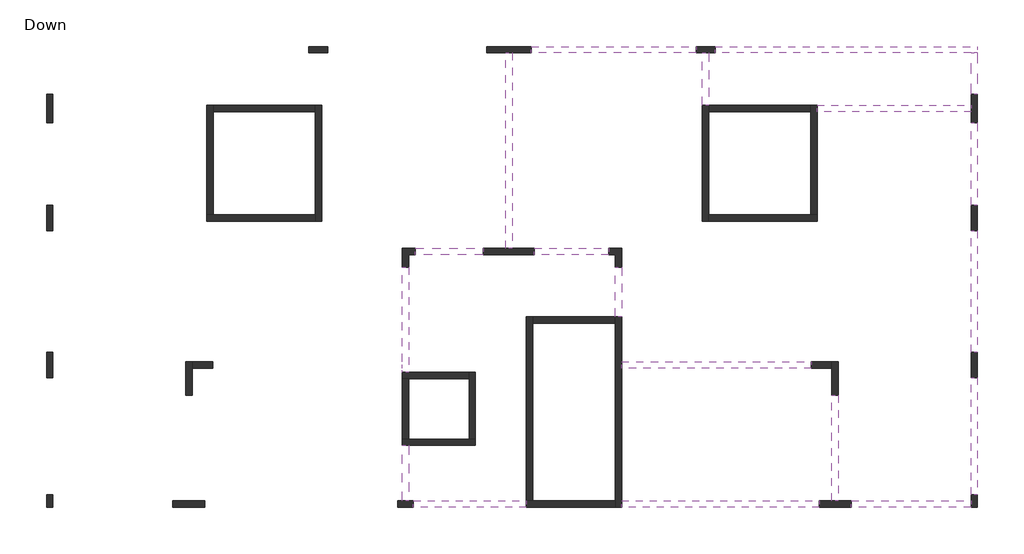
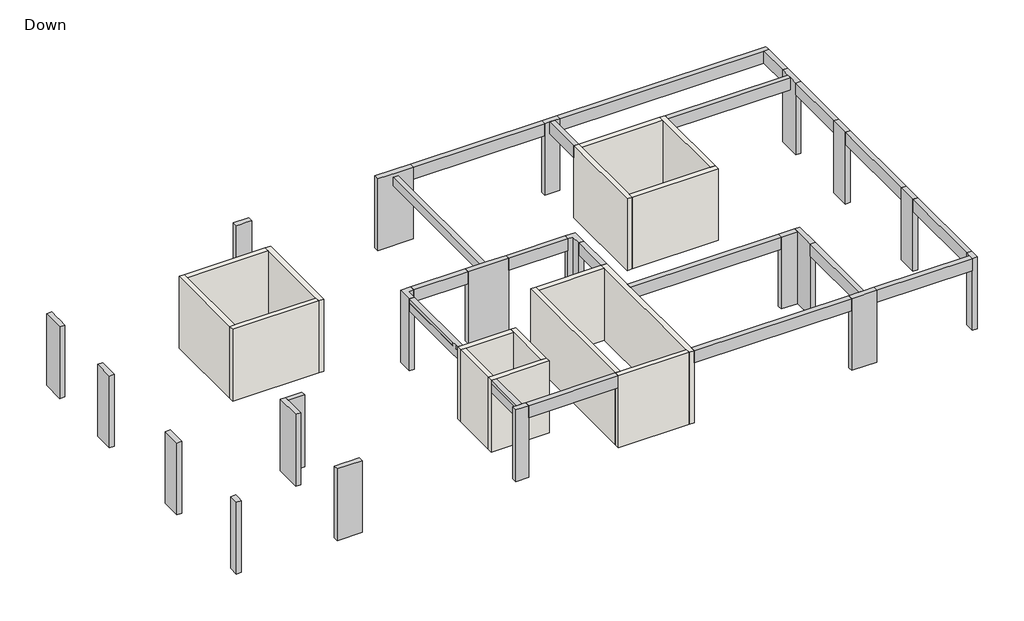
# One storey: 21 columns, 19 beams, 16 walls.
"""IFC4 building model written with IfcOpenShell, lengths in millimetres."""

from ifc_helpers import new_model, si_unit, frame, origin, origin_with_axes, place, context, project, spatial, polyline, outline, extrude, faceted_brep, element, save

model = new_model("IFC4")

# Units and contexts
model_context = context("Model", 3, world=origin())
ifc_project = project(units=[si_unit("LENGTHUNIT", "METRE", prefix="MILLI")], contexts=[model_context])

# Site, building, storey
site = spatial("IfcSite", under=ifc_project)
building = spatial("IfcBuilding", under=site)
storey = spatial("IfcBuildingStorey", under=building, Name="Down", Elevation=0.0)

# Beams
placement = place(None, origin())
element("IfcBeam", 1, ObjectType="Concrete Rectengular Beam : 20/50", at=placement, inside=storey, context=model_context, shape_type="SweptSolid", body=[
    extrude(outline(polyline([(2291.0419081, 4382.4555068), (2291.0419081, 4182.4555068), (-2903.3703529, 4182.4555068), (-2903.3703529, 4382.4555068), (2291.0419081, 4382.4555068)])), frame((0.0, 0.0, 2500.0), z_axis=(0.0, 0.0, 1.0), x_axis=(1.0, 0.0, 0.0)), (0.0, 0.0, 1.0), 500.0),
])
element("IfcBeam", 2, ObjectType="Concrete Rectengular Beam : 20/50", at=placement, inside=storey, context=model_context, shape_type="Brep", body=[
    faceted_brep([(11143.8737416, 4182.4555068, 3000.0), (11143.8737416, 4382.4555068, 3000.0), (2891.0419081, 4382.4555068, 3000.0), (2891.0419081, 4182.4555068, 3000.0), (10943.8737416, 4182.4555068, 3000.0), (11143.8737416, 4182.4555068, 2500.0), (2891.0419081, 4182.4555068, 2500.0), (10943.8737416, 4182.4555068, 2500.0), (11143.8737416, 4382.4555068, 2500.0), (2891.0419081, 4382.4555068, 2500.0)], [[[0, 1, 2, 3, 4]], [[5, 0, 4, 3, 6, 7]], [[8, 5, 7, 6, 9]], [[1, 8, 9, 2]], [[3, 2, 9, 6]], [[1, 0, 5, 8]]]),
])
element("IfcBeam", 3, ObjectType="Concrete Rectengular Beam : 20/50", at=placement, inside=storey, context=model_context, shape_type="Brep", body=[
    faceted_brep([(10943.8737416, 2884.276373, 3000.0), (11143.8737416, 2884.276373, 3000.0), (11143.8737416, 4182.4555068, 3000.0), (10943.8737416, 4182.4555068, 3000.0), (10943.8737416, 2884.276373, 2500.0), (10943.8737416, 4182.4555068, 2850.0), (10943.8737416, 4182.4555068, 2500.0), (11143.8737416, 2884.276373, 2500.0), (11143.8737416, 4182.4555068, 2500.0)], [[[0, 1, 2, 3]], [[4, 0, 3, 5, 6]], [[7, 4, 6, 8]], [[1, 7, 8, 2]], [[1, 0, 4, 7]], [[3, 2, 8, 6, 5]]]),
])
element("IfcBeam", 4, ObjectType="Concrete Rectengular Beam : 20/50", at=placement, inside=storey, context=model_context, shape_type="SweptSolid", body=[
    extrude(outline(polyline([(11143.8737416, -618.260185), (10943.8737416, -618.260185), (10943.8737416, 1984.276373), (11143.8737416, 1984.276373), (11143.8737416, -618.260185)])), frame((0.0, 0.0, 2500.0), z_axis=(0.0, 0.0, 1.0), x_axis=(1.0, 0.0, 0.0)), (0.0, 0.0, 1.0), 500.0),
])
element("IfcBeam", 5, ObjectType="Concrete Rectengular Beam : 20/50", at=placement, inside=storey, context=model_context, shape_type="SweptSolid", body=[
    extrude(outline(polyline([(10943.8737416, -1418.260185), (11143.8737416, -1418.260185), (11143.8737416, -5238.12942), (10943.8737416, -5238.12942), (10943.8737416, -1418.260185)])), frame((0.0, 0.0, 2500.0), z_axis=(0.0, 0.0, 1.0), x_axis=(1.0, 0.0, 0.0)), (0.0, 0.0, 1.0), 500.0),
])
element("IfcBeam", 6, ObjectType="Concrete Rectengular Beam : 20/50", at=placement, inside=storey, context=model_context, shape_type="SweptSolid", body=[
    extrude(outline(polyline([(10943.8737416, -6038.12942), (11143.8737416, -6038.12942), (11143.8737416, -9718.1209836), (10943.8737416, -9718.1209836), (10943.8737416, -6038.12942)])), frame((0.0, 0.0, 2500.0), z_axis=(0.0, 0.0, 1.0), x_axis=(1.0, 0.0, 0.0)), (0.0, 0.0, 1.0), 500.0),
])
element("IfcBeam", 7, ObjectType="Concrete Rectengular Beam : 20/50", at=placement, inside=storey, context=model_context, shape_type="Brep", body=[
    faceted_brep([(5915.4871367, -5738.12942, 3000.0), (5915.4871367, -5538.12942, 3000.0), (-55.6186656, -5538.12942, 3000.0), (-55.6186656, -5738.12942, 3000.0), (5915.4871367, -5538.12942, 2850.0), (5915.4871367, -5538.12942, 2500.0), (-55.6186656, -5538.12942, 2500.0), (-55.6186656, -5538.12942, 2850.0), (5915.4871367, -5738.12942, 2500.0), (-55.6186656, -5738.12942, 2500.0), (-55.6186656, -5738.12942, 2850.0)], [[[0, 1, 2, 3]], [[2, 1, 4, 5, 6, 7]], [[5, 8, 9, 6]], [[8, 0, 3, 10, 9]], [[1, 0, 8, 5, 4]], [[3, 2, 7, 6, 9, 10]]]),
])
element("IfcBeam", 8, ObjectType="Concrete Rectengular Beam : 20/50", at=placement, inside=storey, context=model_context, shape_type="Brep", body=[
    faceted_brep([(6565.4871367, -9918.1209836, 3000.0), (6765.4871367, -9918.1209836, 3000.0), (6765.4871367, -6588.12942, 3000.0), (6565.4871367, -6588.12942, 3000.0), (6565.4871367, -9918.1209836, 2500.0), (6565.4871367, -9918.1209836, 2850.0), (6565.4871367, -6588.12942, 2500.0), (6765.4871367, -9918.1209836, 2500.0), (6765.4871367, -6588.12942, 2500.0), (6765.4871367, -9918.1209836, 2850.0), (6765.4871367, -6588.12942, 2850.0)], [[[0, 1, 2, 3]], [[4, 5, 0, 3, 6]], [[7, 4, 6, 8]], [[2, 1, 9, 7, 8, 10]], [[1, 0, 5, 4, 7, 9]], [[3, 2, 10, 8, 6]]]),
])
element("IfcBeam", 9, ObjectType="Concrete Rectengular Beam : 20/50", at=placement, inside=storey, context=model_context, shape_type="Brep", body=[
    faceted_brep([(10943.8737416, -10118.1209836, 3000.0), (10943.8737416, -9918.1209836, 3000.0), (7164.7300408, -9918.1209836, 3000.0), (7164.7300408, -10118.1209836, 3000.0), (10943.8737416, -10118.1209836, 2500.0), (7164.7300408, -10118.1209836, 2500.0), (10943.8737416, -9918.1209836, 2500.0), (7164.7300408, -9918.1209836, 2500.0), (10943.8737416, -9918.1209836, 2850.0)], [[[0, 1, 2, 3]], [[4, 0, 3, 5]], [[6, 4, 5, 7]], [[1, 8, 6, 7, 2]], [[6, 8, 1, 0, 4]], [[3, 2, 7, 5]]]),
])
element("IfcBeam", 10, ObjectType="Concrete Rectengular Beam : 20/50", at=placement, inside=storey, context=model_context, shape_type="Brep", body=[
    faceted_brep([(10943.8737416, 2334.276373, 3000.0), (10943.8737416, 2534.276373, 3000.0), (6097.3383085, 2534.276373, 3000.0), (6097.3383085, 2334.276373, 3000.0), (10943.8737416, 2534.276373, 2850.0), (10943.8737416, 2534.276373, 2500.0), (6097.3383085, 2534.276373, 2500.0), (10943.8737416, 2334.276373, 2500.0), (6097.3383085, 2334.276373, 2500.0), (6097.3383085, 2334.276373, 2850.0), (10943.8737416, 2334.276373, 2850.0)], [[[0, 1, 2, 3]], [[1, 4, 5, 6, 2]], [[5, 7, 8, 6]], [[0, 3, 9, 8, 7, 10]], [[5, 4, 1, 0, 10, 7]], [[3, 2, 6, 8, 9]]]),
])
element("IfcBeam", 11, ObjectType="Concrete Rectengular Beam : 20/50", at=placement, inside=storey, context=model_context, shape_type="Brep", body=[
    faceted_brep([(2691.0419081, 4182.4555068, 3000.0), (2491.0419081, 4182.4555068, 3000.0), (2491.0419081, 2534.276373, 3000.0), (2691.0419081, 2534.276373, 3000.0), (2491.0419081, 4182.4555068, 2850.0), (2491.0419081, 4182.4555068, 2500.0), (2491.0419081, 2534.276373, 2500.0), (2491.0419081, 2534.276373, 2850.0), (2691.0419081, 4182.4555068, 2500.0), (2691.0419081, 2534.276373, 2500.0), (2691.0419081, 4182.4555068, 2850.0), (2691.0419081, 2534.276373, 2850.0)], [[[0, 1, 2, 3]], [[2, 1, 4, 5, 6, 7]], [[5, 8, 9, 6]], [[8, 10, 0, 3, 11, 9]], [[0, 10, 8, 5, 4, 1]], [[3, 2, 7, 6, 9, 11]]]),
])
element("IfcBeam", 12, ObjectType="Concrete Rectengular Beam : 20/50", at=placement, inside=storey, context=model_context, shape_type="SweptSolid", body=[
    extrude(outline(polyline([(-3703.3703529, 4182.4555068), (-3503.3703529, 4182.4555068), (-3503.3703529, -1968.3192401), (-3703.3703529, -1968.3192401), (-3703.3703529, 4182.4555068)])), frame((0.0, 0.0, 2500.0), z_axis=(0.0, 0.0, 1.0), x_axis=(1.0, 0.0, 0.0)), (0.0, 0.0, 1.0), 350.0),
])
element("IfcBeam", 13, ObjectType="Concrete Rectengular Beam : 20/50", at=placement, inside=storey, context=model_context, shape_type="Brep", body=[
    faceted_brep([(-2804.4614665, -1968.3192401, 3000.0), (-2804.4614665, -2168.3192401, 3000.0), (-455.6186656, -2168.3192401, 3000.0), (-455.6186656, -1968.3192401, 3000.0), (-2804.4614665, -2168.3192401, 2500.0), (-455.6186656, -2168.3192401, 2500.0), (-2804.4614665, -1968.3192401, 2500.0), (-455.6186656, -1968.3192401, 2500.0), (-455.6186656, -1968.3192401, 2850.0), (-2804.4614665, -1968.3192401, 2850.0)], [[[0, 1, 2, 3]], [[1, 4, 5, 2]], [[4, 6, 7, 5]], [[0, 3, 8, 7, 6, 9]], [[1, 0, 9, 6, 4]], [[3, 2, 5, 7, 8]]]),
])
element("IfcBeam", 14, ObjectType="Concrete Rectengular Beam : 20/50", at=placement, inside=storey, context=model_context, shape_type="Brep", body=[
    faceted_brep([(-55.6186656, -2568.3192401, 3000.0), (-255.6186656, -2568.3192401, 3000.0), (-255.6186656, -4117.6485427, 3000.0), (-55.6186656, -4117.6485427, 3000.0), (-255.6186656, -2568.3192401, 2500.0), (-255.6186656, -4117.6485427, 2500.0), (-255.6186656, -4117.6485427, 2850.0), (-55.6186656, -2568.3192401, 2500.0), (-55.6186656, -4117.6485427, 2500.0), (-55.6186656, -4117.6485427, 2850.0), (-55.6186656, -2568.3192401, 2850.0)], [[[0, 1, 2, 3]], [[1, 4, 5, 6, 2]], [[4, 7, 8, 5]], [[0, 3, 9, 8, 7, 10]], [[1, 0, 10, 7, 4]], [[3, 2, 6, 5, 8, 9]]]),
])
element("IfcBeam", 15, ObjectType="Concrete Rectengular Beam : 20/50", at=placement, inside=storey, context=model_context, shape_type="Brep", body=[
    faceted_brep([(6164.7300408, -10118.1209836, 3000.0), (6164.7300408, -9918.1209836, 3000.0), (-55.6186656, -9918.1209836, 3000.0), (-55.6186656, -10118.1209836, 3000.0), (6164.7300408, -9918.1209836, 2500.0), (-55.6186656, -9918.1209836, 2500.0), (-55.6186656, -9918.1209836, 2850.0), (6164.7300408, -10118.1209836, 2500.0), (-55.6186656, -10118.1209836, 2500.0)], [[[0, 1, 2, 3]], [[1, 4, 5, 6, 2]], [[4, 7, 8, 5]], [[7, 0, 3, 8]], [[1, 0, 7, 4]], [[3, 2, 6, 5, 8]]]),
])
element("IfcBeam", 16, ObjectType="Concrete Rectengular Beam : 20/50", at=placement, inside=storey, context=model_context, shape_type="Brep", body=[
    faceted_brep([(-6604.2111853, -9918.1209836, 3000.0), (-6604.2111853, -10118.1209836, 3000.0), (-3055.8548861, -10118.1209836, 3000.0), (-3055.8548861, -9918.1209836, 3000.0), (-6604.2111853, -10118.1209836, 2500.0), (-3055.8548861, -10118.1209836, 2500.0), (-6604.2111853, -9918.1209836, 2500.0), (-3055.8548861, -9918.1209836, 2500.0), (-3055.8548861, -9918.1209836, 2850.0)], [[[0, 1, 2, 3]], [[1, 4, 5, 2]], [[4, 6, 7, 5]], [[6, 0, 3, 8, 7]], [[1, 0, 6, 4]], [[3, 2, 5, 7, 8]]]),
])
element("IfcBeam", 17, ObjectType="Concrete Rectengular Beam : 20/50", at=placement, inside=storey, context=model_context, shape_type="Brep", body=[
    faceted_brep([(-6754.8818827, -9918.1209836, 3000.0), (-6754.8818827, -8168.791681, 3000.0), (-6953.6220402, -8168.791681, 3000.0), (-6953.6220402, -9918.1209836, 3000.0), (-6754.8818827, -9918.1209836, 2850.0), (-6754.8818827, -9918.1209836, 2500.0), (-6754.8818827, -8168.791681, 2500.0), (-6754.8818827, -8168.791681, 2850.0), (-6954.8818827, -9918.1209836, 2500.0), (-6954.8818827, -8168.791681, 2500.0), (-6954.8818827, -9918.1209836, 2850.0), (-6954.8818827, -8168.791681, 2850.0), (-6953.6220402, -9918.1209836, 2850.0), (-6953.6220402, -8168.791681, 2850.0)], [[[0, 1, 2, 3]], [[0, 4, 5, 6, 7, 1]], [[5, 8, 9, 6]], [[9, 8, 10, 11]], [[5, 4, 0, 3, 12, 10, 8]], [[1, 7, 6, 9, 11, 13, 2]], [[12, 13, 11, 10]], [[13, 12, 3, 2]]]),
])
element("IfcBeam", 18, ObjectType="Concrete Rectengular Beam : 20/50", at=placement, inside=storey, context=model_context, shape_type="Brep", body=[
    faceted_brep([(-4404.4614665, -2168.3192401, 3000.0), (-4404.4614665, -1968.3192401, 3000.0), (-6554.5134912, -1968.3192401, 3000.0), (-6554.5134912, -2168.3192401, 3000.0), (-4404.4614665, -1968.3192401, 2850.0), (-4404.4614665, -1968.3192401, 2500.0), (-6554.5134912, -1968.3192401, 2500.0), (-6554.5134912, -1968.3192401, 2850.0), (-4404.4614665, -2168.3192401, 2500.0), (-6554.5134912, -2168.3192401, 2500.0)], [[[0, 1, 2, 3]], [[2, 1, 4, 5, 6, 7]], [[5, 8, 9, 6]], [[8, 0, 3, 9]], [[1, 0, 8, 5, 4]], [[3, 2, 7, 6, 9]]]),
])
element("IfcBeam", 19, ObjectType="Concrete Rectengular Beam : 20/50", at=placement, inside=storey, context=model_context, shape_type="Brep", body=[
    faceted_brep([(-6754.5134912, -5869.1600725, 3000.0), (-6754.5134912, -2568.3192401, 3000.0), (-6951.1220402, -2568.3192401, 3000.0), (-6951.1220402, -5538.12942, 3000.0), (-6954.5134912, -5538.12942, 3000.0), (-6954.5134912, -5738.12942, 3000.0), (-6953.6220402, -5738.12942, 3000.0), (-6953.6220402, -5869.1600725, 3000.0), (-6954.5134912, -2568.3192401, 2500.0), (-6954.5134912, -5538.12942, 2500.0), (-6954.5134912, -5738.12942, 2500.0), (-6954.5134912, -5869.1600725, 2500.0), (-6954.5134912, -5869.1600725, 2850.0), (-6954.5134912, -5738.12942, 2850.0), (-6954.5134912, -5538.12942, 2850.0), (-6954.5134912, -2568.3192401, 2850.0), (-6754.5134912, -2568.3192401, 2500.0), (-6754.5134912, -5869.1600725, 2500.0), (-6754.5134912, -5869.1600725, 2850.0), (-6754.5134912, -2568.3192401, 2850.0), (-6951.1220402, -2568.3192401, 2850.0), (-6953.6220402, -5869.1600725, 2850.0), (-6953.6220402, -5738.12942, 2850.0), (-6951.1220402, -5538.12942, 2850.0)], [[[0, 1, 2, 3, 4, 5, 6, 7]], [[8, 9, 10, 11, 12, 13, 5, 4, 14, 15]], [[8, 16, 17, 11, 10, 9]], [[1, 0, 18, 17, 16, 19]], [[16, 8, 15, 20, 2, 1, 19]], [[11, 17, 18, 0, 7, 21, 12]], [[21, 22, 13, 12]], [[6, 22, 21, 7]], [[22, 6, 5, 13]], [[14, 23, 20, 15]], [[3, 23, 14, 4]], [[23, 3, 2, 20]]]),
])

# Columns
element("IfcColumn", 20, ObjectType="Concrete Rectengular Column : 20/100", at=placement, inside=storey, context=model_context, shape_type="Brep", body=[
    faceted_brep([(6164.7300408, -9918.1209836, 0.0), (7164.7300408, -9918.1209836, 0.0), (7164.7300408, -10118.1209836, 0.0), (6164.7300408, -10118.1209836, 0.0), (6164.7300408, -9918.1209836, 3000.0), (6565.4871367, -9918.1209836, 3000.0), (6765.4871367, -9918.1209836, 3000.0), (7164.7300408, -9918.1209836, 3000.0), (7164.7300408, -10118.1209836, 3000.0), (6164.7300408, -10118.1209836, 3000.0)], [[[0, 1, 2, 3]], [[4, 5, 6, 7, 1, 0]], [[7, 8, 2, 1]], [[8, 9, 3, 2]], [[9, 4, 0, 3]], [[4, 9, 8, 7, 6, 5]]]),
])
element("IfcColumn", 21, ObjectType="Concrete Rectengular Column : 20/100", at=placement, inside=storey, context=model_context, shape_type="Brep", body=[
    faceted_brep([(-13171.4707466, -9918.1209836, 0.0), (-13171.4707466, -10118.1209836, 0.0), (-14171.4707466, -10118.1209836, 0.0), (-14171.4707466, -9918.1209836, 0.0), (-13171.4707466, -9918.1209836, 3000.0), (-14171.4707466, -9918.1209836, 3000.0), (-13772.2278424, -9918.1209836, 3000.0), (-13572.2278424, -9918.1209836, 3000.0), (-14171.4707466, -10118.1209836, 3000.0), (-13171.4707466, -10118.1209836, 3000.0)], [[[0, 1, 2, 3]], [[4, 0, 3, 5, 6, 7]], [[5, 3, 2, 8]], [[8, 2, 1, 9]], [[9, 1, 0, 4]], [[4, 7, 6, 5, 8, 9]]]),
])
element("IfcColumn", 22, ObjectType="Concrete Rectengular Column : 20/105", at=placement, inside=storey, context=model_context, shape_type="Brep", body=[
    faceted_brep([(6765.4871367, -5538.12942, 0.0), (6765.4871367, -6588.12942, 0.0), (6565.4871367, -6588.12942, 0.0), (6565.4871367, -5738.12942, 0.0), (6565.4871367, -5538.12942, 0.0), (6765.4871367, -5538.12942, 3000.0), (6765.4871367, -6588.12942, 3000.0), (6765.4871367, -5538.12942, 2850.0), (6565.4871367, -6588.12942, 3000.0), (6565.4871367, -5738.12942, 3000.0), (6565.4871367, -5538.12942, 3000.0)], [[[0, 1, 2, 3, 4]], [[5, 6, 1, 0, 7]], [[6, 8, 2, 1]], [[8, 9, 10, 4, 3, 2]], [[10, 5, 7, 0, 4]], [[5, 10, 9, 8, 6]]]),
])
element("IfcColumn", 23, ObjectType="Concrete Rectengular Column : 20/105", at=placement, inside=storey, context=model_context, shape_type="Brep", body=[
    faceted_brep([(-13772.2278424, -5538.12942, 0.0), (-13572.2278424, -5538.12942, 0.0), (-13572.2278424, -5738.12942, 0.0), (-13572.2278424, -6588.12942, 0.0), (-13772.2278424, -6588.12942, 0.0), (-13772.2278424, -5538.12942, 3000.0), (-13772.2278424, -5538.12942, 2850.0), (-13772.2278424, -6588.12942, 3000.0), (-13572.2278424, -6588.12942, 3000.0), (-13572.2278424, -5538.12942, 3000.0), (-13572.2278424, -5738.12942, 3000.0)], [[[0, 1, 2, 3, 4]], [[5, 6, 0, 4, 7]], [[7, 4, 3, 8]], [[8, 3, 2, 1, 9, 10]], [[9, 1, 0, 6, 5]], [[5, 7, 8, 10, 9]]]),
])
element("IfcColumn", 24, ObjectType="Concrete Rectengular Column : 20/140", at=placement, inside=storey, context=model_context, shape_type="Brep", body=[
    faceted_brep([(-4303.3703529, 4382.4555068, 0.0), (-2903.3703529, 4382.4555068, 0.0), (-2903.3703529, 4182.4555068, 0.0), (-4303.3703529, 4182.4555068, 0.0), (-4303.3703529, 4382.4555068, 3000.0), (-2903.3703529, 4382.4555068, 3000.0), (-2903.3703529, 4182.4555068, 3000.0), (-3503.3703529, 4182.4555068, 3000.0), (-4303.3703529, 4182.4555068, 3000.0)], [[[0, 1, 2, 3]], [[4, 5, 1, 0]], [[5, 6, 2, 1]], [[6, 7, 8, 3, 2]], [[8, 4, 0, 3]], [[4, 8, 7, 6, 5]]]),
])
element("IfcColumn", 25, ObjectType="Concrete Rectengular Column : 20/160", at=placement, inside=storey, context=model_context, shape_type="Brep", body=[
    faceted_brep([(-4404.4614665, -1968.3192401, 0.0), (-2804.4614665, -1968.3192401, 0.0), (-2804.4614665, -2168.3192401, 0.0), (-4404.4614665, -2168.3192401, 0.0), (-4404.4614665, -1968.3192401, 3000.0), (-3503.3703529, -1968.3192401, 3000.0), (-2804.4614665, -1968.3192401, 3000.0), (-2804.4614665, -2168.3192401, 3000.0), (-4404.4614665, -2168.3192401, 3000.0)], [[[0, 1, 2, 3]], [[4, 5, 6, 1, 0]], [[6, 7, 2, 1]], [[7, 8, 3, 2]], [[8, 4, 0, 3]], [[4, 8, 7, 6, 5]]]),
])
element("IfcColumn", 26, ObjectType="Concrete Rectengular Column : 20/40", at=placement, inside=storey, context=model_context, shape_type="Brep", body=[
    faceted_brep([(11143.8737416, -9718.1209836, 0.0), (11143.8737416, -10118.1209836, 0.0), (10943.8737416, -10118.1209836, 0.0), (10943.8737416, -9718.1209836, 0.0), (11143.8737416, -9718.1209836, 3000.0), (11143.8737416, -10118.1209836, 3000.0), (10943.8737416, -10118.1209836, 3000.0), (10943.8737416, -9918.1209836, 3000.0), (10943.8737416, -9718.1209836, 3000.0)], [[[0, 1, 2, 3]], [[4, 5, 1, 0]], [[5, 6, 2, 1]], [[6, 7, 8, 3, 2]], [[8, 4, 0, 3]], [[4, 8, 7, 6, 5]]]),
])
element("IfcColumn", 27, ObjectType="Concrete Rectengular Column : 20/40", at=placement, inside=storey, context=model_context, shape_type="Brep", body=[
    faceted_brep([(-18150.6144474, -9718.1209836, 0.0), (-17950.6144474, -9718.1209836, 0.0), (-17950.6144474, -10118.1209836, 0.0), (-18150.6144474, -10118.1209836, 0.0), (-18150.6144474, -9718.1209836, 3000.0), (-18150.6144474, -10118.1209836, 3000.0), (-17950.6144474, -10118.1209836, 3000.0), (-17950.6144474, -9718.1209836, 3000.0), (-17950.6144474, -9918.1209836, 3000.0)], [[[0, 1, 2, 3]], [[4, 0, 3, 5]], [[5, 3, 2, 6]], [[6, 2, 1, 7, 8]], [[7, 1, 0, 4]], [[4, 5, 6, 8, 7]]]),
])
element("IfcColumn", 28, ObjectType="Concrete Rectengular Column : 20/50", at=placement, inside=storey, context=model_context, shape_type="Brep", body=[
    faceted_brep([(-7104.2111853, -9918.1209836, 0.0), (-6604.2111853, -9918.1209836, 0.0), (-6604.2111853, -10118.1209836, 0.0), (-7104.2111853, -10118.1209836, 0.0), (-7104.2111853, -9918.1209836, 3000.0), (-6953.6220402, -9918.1209836, 3000.0), (-6754.8818827, -9918.1209836, 3000.0), (-6604.2111853, -9918.1209836, 3000.0), (-6604.2111853, -10118.1209836, 3000.0), (-7104.2111853, -10118.1209836, 3000.0)], [[[0, 1, 2, 3]], [[4, 5, 6, 7, 1, 0]], [[7, 8, 2, 1]], [[8, 9, 3, 2]], [[9, 4, 0, 3]], [[4, 9, 8, 7, 6, 5]]]),
])
element("IfcColumn", 29, ObjectType="Concrete Rectengular Column : 20/60", at=placement, inside=storey, context=model_context, shape_type="Brep", body=[
    faceted_brep([(2291.0419081, 4382.4555068, 0.0), (2891.0419081, 4382.4555068, 0.0), (2891.0419081, 4182.4555068, 0.0), (2291.0419081, 4182.4555068, 0.0), (2291.0419081, 4382.4555068, 3000.0), (2891.0419081, 4382.4555068, 3000.0), (2891.0419081, 4182.4555068, 3000.0), (2691.0419081, 4182.4555068, 3000.0), (2491.0419081, 4182.4555068, 3000.0), (2291.0419081, 4182.4555068, 3000.0)], [[[0, 1, 2, 3]], [[4, 5, 1, 0]], [[5, 6, 2, 1]], [[6, 7, 8, 9, 3, 2]], [[9, 4, 0, 3]], [[4, 9, 8, 7, 6, 5]]]),
])
element("IfcColumn", 30, ObjectType="Concrete Rectengular Column : 20/60", at=placement, inside=storey, context=model_context, shape_type="Brep", body=[
    faceted_brep([(-9297.7826138, 4382.4555068, 0.0), (-9297.7826138, 4182.4555068, 0.0), (-9897.7826138, 4182.4555068, 0.0), (-9897.7826138, 4382.4555068, 0.0), (-9297.7826138, 4382.4555068, 3000.0), (-9897.7826138, 4382.4555068, 3000.0), (-9897.7826138, 4182.4555068, 3000.0), (-9297.7826138, 4182.4555068, 3000.0), (-9497.7826138, 4182.4555068, 3000.0), (-9697.7826138, 4182.4555068, 3000.0)], [[[0, 1, 2, 3]], [[4, 0, 3, 5]], [[5, 3, 2, 6]], [[6, 2, 1, 7, 8, 9]], [[7, 1, 0, 4]], [[4, 5, 6, 9, 8, 7]]]),
])
element("IfcColumn", 31, ObjectType="Concrete Rectengular Column : 20/65", at=placement, inside=storey, context=model_context, shape_type="Brep", body=[
    faceted_brep([(5915.4871367, -5538.12942, 0.0), (6565.4871367, -5538.12942, 0.0), (6565.4871367, -5738.12942, 0.0), (5915.4871367, -5738.12942, 0.0), (5915.4871367, -5538.12942, 3000.0), (6565.4871367, -5538.12942, 3000.0), (6565.4871367, -5738.12942, 3000.0), (6565.4871367, -5738.12942, 2850.0), (5915.4871367, -5738.12942, 3000.0)], [[[0, 1, 2, 3]], [[4, 5, 1, 0]], [[5, 6, 7, 2, 1]], [[6, 8, 3, 2, 7]], [[8, 4, 0, 3]], [[4, 8, 6, 5]]]),
])
element("IfcColumn", 32, ObjectType="Concrete Rectengular Column : 20/65", at=placement, inside=storey, context=model_context, shape_type="Brep", body=[
    faceted_brep([(-12922.2278424, -5538.12942, 0.0), (-12922.2278424, -5738.12942, 0.0), (-13572.2278424, -5738.12942, 0.0), (-13572.2278424, -5538.12942, 0.0), (-12922.2278424, -5538.12942, 3000.0), (-13572.2278424, -5538.12942, 3000.0), (-13572.2278424, -5738.12942, 2850.0), (-13572.2278424, -5738.12942, 3000.0), (-12922.2278424, -5738.12942, 3000.0)], [[[0, 1, 2, 3]], [[4, 0, 3, 5]], [[5, 3, 2, 6, 7]], [[7, 6, 2, 1, 8]], [[8, 1, 0, 4]], [[4, 5, 7, 8]]]),
])
element("IfcColumn", 33, ObjectType="Concrete Rectengular Column : 20/80", at=placement, inside=storey, context=model_context, shape_type="SweptSolid", body=[
    extrude(outline(polyline([(11143.8737416, -618.260185), (11143.8737416, -1418.260185), (10943.8737416, -1418.260185), (10943.8737416, -618.260185), (11143.8737416, -618.260185)])), origin_with_axes(), (0.0, 0.0, 1.0), 3000.0),
])
element("IfcColumn", 34, ObjectType="Concrete Rectengular Column : 20/80", at=placement, inside=storey, context=model_context, shape_type="SweptSolid", body=[
    extrude(outline(polyline([(11143.8737416, -5238.12942), (11143.8737416, -6038.12942), (10943.8737416, -6038.12942), (10943.8737416, -5238.12942), (11143.8737416, -5238.12942)])), origin_with_axes(), (0.0, 0.0, 1.0), 3000.0),
])
element("IfcColumn", 35, ObjectType="Concrete Rectengular Column : 20/80", at=placement, inside=storey, context=model_context, shape_type="SweptSolid", body=[
    extrude(outline(polyline([(-18150.6144474, -618.260185), (-17950.6144474, -618.260185), (-17950.6144474, -1418.260185), (-18150.6144474, -1418.260185), (-18150.6144474, -618.260185)])), origin_with_axes(), (0.0, 0.0, 1.0), 3000.0),
])
element("IfcColumn", 36, ObjectType="Concrete Rectengular Column : 20/80", at=placement, inside=storey, context=model_context, shape_type="SweptSolid", body=[
    extrude(outline(polyline([(-18150.6144474, -5238.12942), (-17950.6144474, -5238.12942), (-17950.6144474, -6038.12942), (-18150.6144474, -6038.12942), (-18150.6144474, -5238.12942)])), origin_with_axes(), (0.0, 0.0, 1.0), 3000.0),
])
element("IfcColumn", 37, ObjectType="Concrete Rectengular Column : 20/90", at=placement, inside=storey, context=model_context, shape_type="Brep", body=[
    faceted_brep([(11143.8737416, 2884.276373, 0.0), (11143.8737416, 1984.276373, 0.0), (10943.8737416, 1984.276373, 0.0), (10943.8737416, 2884.276373, 0.0), (11143.8737416, 2884.276373, 3000.0), (11143.8737416, 1984.276373, 3000.0), (10943.8737416, 1984.276373, 3000.0), (10943.8737416, 2334.276373, 3000.0), (10943.8737416, 2534.276373, 3000.0), (10943.8737416, 2884.276373, 3000.0)], [[[0, 1, 2, 3]], [[4, 5, 1, 0]], [[5, 6, 2, 1]], [[6, 7, 8, 9, 3, 2]], [[9, 4, 0, 3]], [[4, 9, 8, 7, 6, 5]]]),
])
element("IfcColumn", 38, ObjectType="Concrete Rectengular Column : 20/90", at=placement, inside=storey, context=model_context, shape_type="Brep", body=[
    faceted_brep([(-18150.6144474, 2884.276373, 0.0), (-17950.6144474, 2884.276373, 0.0), (-17950.6144474, 1984.276373, 0.0), (-18150.6144474, 1984.276373, 0.0), (-18150.6144474, 2884.276373, 3000.0), (-18150.6144474, 1984.276373, 3000.0), (-17950.6144474, 1984.276373, 3000.0), (-17950.6144474, 2884.276373, 3000.0), (-17950.6144474, 2534.276373, 3000.0), (-17950.6144474, 2334.276373, 3000.0)], [[[0, 1, 2, 3]], [[4, 0, 3, 5]], [[5, 3, 2, 6]], [[6, 2, 1, 7, 8, 9]], [[7, 1, 0, 4]], [[4, 5, 6, 9, 8, 7]]]),
])
element("IfcColumn", 39, ObjectType="L Column : 20/40/20/20", at=placement, inside=storey, context=model_context, shape_type="Brep", body=[
    faceted_brep([(-6954.5134912, -1968.3192401, 0.0), (-6554.5134912, -1968.3192401, 0.0), (-6554.5134912, -2168.3192401, 0.0), (-6754.5134912, -2168.3192401, 0.0), (-6754.5134912, -2568.3192401, 0.0), (-6954.5134912, -2568.3192401, 0.0), (-6954.5134912, -1968.3192401, 3000.0), (-6554.5134912, -1968.3192401, 3000.0), (-6954.5134912, -1968.3192401, 2850.0), (-6554.5134912, -2168.3192401, 3000.0), (-6754.5134912, -2168.3192401, 3000.0), (-6754.5134912, -2168.3192401, 2850.0), (-6754.5134912, -2568.3192401, 3000.0), (-6951.1220402, -2568.3192401, 3000.0), (-6954.5134912, -2568.3192401, 3000.0), (-6954.5134912, -2568.3192401, 2850.0)], [[[0, 1, 2, 3, 4, 5]], [[6, 7, 1, 0, 8]], [[7, 9, 2, 1]], [[9, 10, 11, 3, 2]], [[10, 12, 4, 3, 11]], [[12, 13, 14, 15, 5, 4]], [[14, 6, 8, 0, 5, 15]], [[6, 14, 13, 12, 10, 9, 7]]]),
])
element("IfcColumn", 40, ObjectType="L Column : 20/40/20/20", at=placement, inside=storey, context=model_context, shape_type="Brep", body=[
    faceted_brep([(-55.6186656, -1968.3192401, 0.0), (-55.6186656, -2568.3192401, 0.0), (-255.6186656, -2568.3192401, 0.0), (-255.6186656, -2168.3192401, 0.0), (-455.6186656, -2168.3192401, 0.0), (-455.6186656, -1968.3192401, 0.0), (-55.6186656, -1968.3192401, 3000.0), (-55.6186656, -1968.3192401, 2850.0), (-455.6186656, -1968.3192401, 3000.0), (-455.6186656, -2168.3192401, 3000.0), (-255.6186656, -2168.3192401, 2850.0), (-255.6186656, -2168.3192401, 3000.0), (-255.6186656, -2568.3192401, 3000.0), (-55.6186656, -2568.3192401, 3000.0)], [[[0, 1, 2, 3, 4, 5]], [[6, 7, 0, 5, 8]], [[8, 5, 4, 9]], [[9, 4, 3, 10, 11]], [[11, 10, 3, 2, 12]], [[12, 2, 1, 13]], [[13, 1, 0, 7, 6]], [[6, 8, 9, 11, 12, 13]]]),
])

# Walls
element("IfcWall", 41, ObjectType="20", at=placement, inside=storey, context=model_context, shape_type="Brep", body=[
    faceted_brep([(2491.0419081, 2534.276373, 0.0), (2491.0419081, -1117.4123222, 0.0), (2491.0419081, -1117.4123222, 2850.0), (2491.0419081, -1117.4123222, 3000.0), (2491.0419081, 2534.276373, 3000.0), (2491.0419081, 2534.276373, 2500.0), (2691.0419081, 2534.276373, 0.0), (2691.0419081, 2534.276373, 2500.0), (2691.0419081, 2534.276373, 3000.0), (2691.0419081, 2334.276373, 3000.0), (2691.0419081, -917.4123222, 3000.0), (2691.0419081, -1117.4123222, 3000.0), (2691.0419081, -1117.4123222, 0.0), (2691.0419081, -917.4123222, 0.0), (2691.0419081, 2334.276373, 0.0)], [[[0, 1, 2, 3, 4, 5]], [[6, 7, 8, 9, 10, 11, 12, 13, 14]], [[1, 0, 6, 14, 13, 12]], [[4, 3, 11, 10, 9, 8]], [[3, 2, 1, 12, 11]], [[0, 5, 4, 8, 7, 6]]]),
])
element("IfcWall", 42, ObjectType="20", at=placement, inside=storey, context=model_context, shape_type="Brep", body=[
    faceted_brep([(2691.0419081, -1117.4123222, 0.0), (6097.3383085, -1117.4123222, 0.0), (6097.3383085, -1117.4123222, 2850.0), (6097.3383085, -1117.4123222, 3000.0), (2691.0419081, -1117.4123222, 3000.0), (2691.0419081, -917.4123222, 0.0), (2691.0419081, -917.4123222, 2850.0), (2691.0419081, -917.4123222, 3000.0), (5897.3383085, -917.4123222, 3000.0), (6097.3383085, -917.4123222, 3000.0), (6097.3383085, -917.4123222, 0.0), (5897.3383085, -917.4123222, 0.0)], [[[0, 1, 2, 3, 4]], [[5, 6, 7, 8, 9, 10, 11]], [[1, 0, 5, 11, 10]], [[4, 3, 9, 8, 7]], [[0, 4, 7, 6, 5]], [[3, 2, 1, 10, 9]]]),
])
element("IfcWall", 43, ObjectType="20", at=placement, inside=storey, context=model_context, shape_type="Brep", body=[
    faceted_brep([(6097.3383085, -917.4123222, 0.0), (6097.3383085, 2534.276373, 0.0), (6097.3383085, 2534.276373, 3000.0), (6097.3383085, 2334.276373, 3000.0), (6097.3383085, -917.4123222, 3000.0), (5897.3383085, -917.4123222, 0.0), (5897.3383085, -917.4123222, 2850.0), (5897.3383085, -917.4123222, 3000.0), (5897.3383085, 2334.276373, 3000.0), (5897.3383085, 2534.276373, 3000.0), (5897.3383085, 2534.276373, 0.0), (5897.3383085, 2334.276373, 0.0)], [[[0, 1, 2, 3, 4]], [[5, 6, 7, 8, 9, 10, 11]], [[1, 0, 5, 11, 10]], [[4, 3, 2, 9, 8, 7]], [[0, 4, 7, 6, 5]], [[2, 1, 10, 9]]]),
])
element("IfcWall", 44, ObjectType="20", at=placement, inside=storey, context=model_context, shape_type="Brep", body=[
    faceted_brep([(5897.3383085, 2534.276373, 0.0), (2691.0419081, 2534.276373, 0.0), (2691.0419081, 2534.276373, 2850.0), (2691.0419081, 2534.276373, 3000.0), (5897.3383085, 2534.276373, 3000.0), (5897.3383085, 2334.276373, 0.0), (5897.3383085, 2334.276373, 2850.0), (5897.3383085, 2334.276373, 3000.0), (2691.0419081, 2334.276373, 3000.0), (2691.0419081, 2334.276373, 2850.0), (2691.0419081, 2334.276373, 0.0)], [[[0, 1, 2, 3, 4]], [[5, 6, 7, 8, 9, 10]], [[1, 0, 5, 10]], [[4, 3, 8, 7]], [[0, 4, 7, 6, 5]], [[3, 2, 1, 10, 9, 8]]]),
])
element("IfcWall", 45, ObjectType="20", at=placement, inside=storey, context=model_context, shape_type="Brep", body=[
    faceted_brep([(-255.6186656, -4117.6485427, 0.0), (-255.6186656, -4317.6485427, 0.0), (-255.6186656, -9918.1209836, 0.0), (-255.6186656, -10118.1209836, 0.0), (-255.6186656, -10118.1209836, 3000.0), (-255.6186656, -9918.1209836, 3000.0), (-255.6186656, -4317.6485427, 3000.0), (-255.6186656, -4117.6485427, 3000.0), (-255.6186656, -4117.6485427, 2500.0), (-55.6186656, -4117.6485427, 0.0), (-55.6186656, -4117.6485427, 2500.0), (-55.6186656, -4117.6485427, 3000.0), (-55.6186656, -5538.12942, 3000.0), (-55.6186656, -5738.12942, 3000.0), (-55.6186656, -9918.1209836, 3000.0), (-55.6186656, -10118.1209836, 3000.0), (-55.6186656, -10118.1209836, 0.0)], [[[0, 1, 2, 3, 4, 5, 6, 7, 8]], [[9, 10, 11, 12, 13, 14, 15, 16]], [[3, 2, 1, 0, 9, 16]], [[7, 6, 5, 4, 15, 14, 13, 12, 11]], [[4, 3, 16, 15]], [[0, 8, 7, 11, 10, 9]]]),
])
element("IfcWall", 46, ObjectType="20", at=placement, inside=storey, context=model_context, shape_type="Brep", body=[
    faceted_brep([(-255.6186656, -9918.1209836, 0.0), (-2855.8548861, -9918.1209836, 0.0), (-3055.8548861, -9918.1209836, 0.0), (-3055.8548861, -9918.1209836, 2500.0), (-3055.8548861, -9918.1209836, 3000.0), (-2855.8548861, -9918.1209836, 3000.0), (-255.6186656, -9918.1209836, 3000.0), (-255.6186656, -9918.1209836, 2850.0), (-255.6186656, -10118.1209836, 0.0), (-255.6186656, -10118.1209836, 3000.0), (-3055.8548861, -10118.1209836, 3000.0), (-3055.8548861, -10118.1209836, 2500.0), (-3055.8548861, -10118.1209836, 0.0)], [[[0, 1, 2, 3, 4, 5, 6, 7]], [[8, 9, 10, 11, 12]], [[2, 1, 0, 8, 12]], [[6, 5, 4, 10, 9]], [[0, 7, 6, 9, 8]], [[4, 3, 2, 12, 11, 10]]]),
])
element("IfcWall", 47, ObjectType="20", at=placement, inside=storey, context=model_context, shape_type="Brep", body=[
    faceted_brep([(-2855.8548861, -9918.1209836, 0.0), (-2855.8548861, -4317.6485427, 0.0), (-2855.8548861, -4117.6485427, 0.0), (-2855.8548861, -4117.6485427, 3000.0), (-2855.8548861, -4317.6485427, 3000.0), (-2855.8548861, -9918.1209836, 3000.0), (-2855.8548861, -9918.1209836, 2850.0), (-3055.8548861, -9918.1209836, 0.0), (-3055.8548861, -9918.1209836, 2850.0), (-3055.8548861, -9918.1209836, 3000.0), (-3055.8548861, -4117.6485427, 3000.0), (-3055.8548861, -4117.6485427, 2850.0), (-3055.8548861, -4117.6485427, 0.0)], [[[0, 1, 2, 3, 4, 5, 6]], [[7, 8, 9, 10, 11, 12]], [[2, 1, 0, 7, 12]], [[5, 4, 3, 10, 9]], [[0, 6, 5, 9, 8, 7]], [[3, 2, 12, 11, 10]]]),
])
element("IfcWall", 48, ObjectType="20", at=placement, inside=storey, context=model_context, shape_type="Brep", body=[
    faceted_brep([(-2855.8548861, -4317.6485427, 0.0), (-255.6186656, -4317.6485427, 0.0), (-255.6186656, -4317.6485427, 2850.0), (-255.6186656, -4317.6485427, 3000.0), (-2855.8548861, -4317.6485427, 3000.0), (-2855.8548861, -4317.6485427, 2850.0), (-2855.8548861, -4117.6485427, 0.0), (-2855.8548861, -4117.6485427, 3000.0), (-255.6186656, -4117.6485427, 3000.0), (-255.6186656, -4117.6485427, 2850.0), (-255.6186656, -4117.6485427, 0.0)], [[[0, 1, 2, 3, 4, 5]], [[6, 7, 8, 9, 10]], [[1, 0, 6, 10]], [[4, 3, 8, 7]], [[3, 2, 1, 10, 9, 8]], [[0, 5, 4, 7, 6]]]),
])
element("IfcWall", 49, ObjectType="20", at=placement, inside=storey, context=model_context, shape_type="Brep", body=[
    faceted_brep([(-6954.8818827, -8168.791681, 0.0), (-4654.8818827, -8168.791681, 0.0), (-4654.8818827, -8168.791681, 2850.0), (-4654.8818827, -8168.791681, 3000.0), (-6754.8818827, -8168.791681, 3000.0), (-6953.6220402, -8168.791681, 3000.0), (-6954.8818827, -8168.791681, 3000.0), (-6954.8818827, -8168.791681, 2850.0), (-6954.8818827, -7968.791681, 0.0), (-6954.8818827, -7968.791681, 3000.0), (-6754.8818827, -7968.791681, 3000.0), (-4854.8818827, -7968.791681, 3000.0), (-4654.8818827, -7968.791681, 3000.0), (-4654.8818827, -7968.791681, 0.0), (-4854.8818827, -7968.791681, 0.0), (-6754.8818827, -7968.791681, 0.0)], [[[0, 1, 2, 3, 4, 5, 6, 7]], [[8, 9, 10, 11, 12, 13, 14, 15]], [[1, 0, 8, 15, 14, 13]], [[6, 5, 4, 3, 12, 11, 10, 9]], [[3, 2, 1, 13, 12]], [[0, 7, 6, 9, 8]]]),
])
element("IfcWall", 50, ObjectType="20", at=placement, inside=storey, context=model_context, shape_type="Brep", body=[
    faceted_brep([(-4654.8818827, -7968.791681, 0.0), (-4654.8818827, -5869.1600725, 0.0), (-4654.8818827, -5869.1600725, 2850.0), (-4654.8818827, -5869.1600725, 3000.0), (-4654.8818827, -7968.791681, 3000.0), (-4854.8818827, -7968.791681, 0.0), (-4854.8818827, -7968.791681, 2850.0), (-4854.8818827, -7968.791681, 3000.0), (-4854.8818827, -6069.1600725, 3000.0), (-4854.8818827, -5869.1600725, 3000.0), (-4854.8818827, -5869.1600725, 0.0), (-4854.8818827, -6069.1600725, 0.0)], [[[0, 1, 2, 3, 4]], [[5, 6, 7, 8, 9, 10, 11]], [[1, 0, 5, 11, 10]], [[4, 3, 9, 8, 7]], [[0, 4, 7, 6, 5]], [[3, 2, 1, 10, 9]]]),
])
element("IfcWall", 51, ObjectType="20", at=placement, inside=storey, context=model_context, shape_type="Brep", body=[
    faceted_brep([(-4854.8818827, -5869.1600725, 0.0), (-6954.8818827, -5869.1600725, 0.0), (-6954.8818827, -5869.1600725, 2850.0), (-6954.8818827, -5869.1600725, 3000.0), (-6953.6220402, -5869.1600725, 3000.0), (-6754.5134912, -5869.1600725, 3000.0), (-4854.8818827, -5869.1600725, 3000.0), (-4854.8818827, -6069.1600725, 0.0), (-4854.8818827, -6069.1600725, 2850.0), (-4854.8818827, -6069.1600725, 3000.0), (-6754.8818827, -6069.1600725, 3000.0), (-6954.8818827, -6069.1600725, 3000.0), (-6954.8818827, -6069.1600725, 0.0), (-6754.8818827, -6069.1600725, 0.0)], [[[0, 1, 2, 3, 4, 5, 6]], [[7, 8, 9, 10, 11, 12, 13]], [[1, 0, 7, 13, 12]], [[6, 5, 4, 3, 11, 10, 9]], [[0, 6, 9, 8, 7]], [[3, 2, 1, 12, 11]]]),
])
element("IfcWall", 52, ObjectType="20", at=placement, inside=storey, context=model_context, shape_type="Brep", body=[
    faceted_brep([(-6954.8818827, -6069.1600725, 0.0), (-6954.8818827, -7968.791681, 0.0), (-6954.8818827, -7968.791681, 3000.0), (-6954.8818827, -6069.1600725, 3000.0), (-6754.8818827, -6069.1600725, 0.0), (-6754.8818827, -6069.1600725, 2850.0), (-6754.8818827, -6069.1600725, 3000.0), (-6754.8818827, -7968.791681, 3000.0), (-6754.8818827, -7968.791681, 2850.0), (-6754.8818827, -7968.791681, 0.0)], [[[0, 1, 2, 3]], [[4, 5, 6, 7, 8, 9]], [[1, 0, 4, 9]], [[3, 2, 7, 6]], [[0, 3, 6, 5, 4]], [[2, 1, 9, 8, 7]]]),
])
element("IfcWall", 53, ObjectType="20", at=placement, inside=storey, context=model_context, shape_type="Brep", body=[
    faceted_brep([(-9697.7826138, 2534.276373, 0.0), (-9697.7826138, 2334.276373, 0.0), (-9697.7826138, -917.4123222, 0.0), (-9697.7826138, -1117.4123222, 0.0), (-9697.7826138, -1117.4123222, 3000.0), (-9697.7826138, -917.4123222, 3000.0), (-9697.7826138, 2334.276373, 3000.0), (-9697.7826138, 2534.276373, 3000.0), (-9697.7826138, 2534.276373, 2500.0), (-9497.7826138, 2534.276373, 0.0), (-9497.7826138, 2534.276373, 2500.0), (-9497.7826138, 2534.276373, 3000.0), (-9497.7826138, -1117.4123222, 3000.0), (-9497.7826138, -1117.4123222, 2850.0), (-9497.7826138, -1117.4123222, 0.0)], [[[0, 1, 2, 3, 4, 5, 6, 7, 8]], [[9, 10, 11, 12, 13, 14]], [[3, 2, 1, 0, 9, 14]], [[7, 6, 5, 4, 12, 11]], [[4, 3, 14, 13, 12]], [[0, 8, 7, 11, 10, 9]]]),
])
element("IfcWall", 54, ObjectType="20", at=placement, inside=storey, context=model_context, shape_type="Brep", body=[
    faceted_brep([(-9697.7826138, -917.4123222, 0.0), (-12904.0790143, -917.4123222, 0.0), (-13104.0790143, -917.4123222, 0.0), (-13104.0790143, -917.4123222, 3000.0), (-12904.0790143, -917.4123222, 3000.0), (-9697.7826138, -917.4123222, 3000.0), (-9697.7826138, -917.4123222, 2850.0), (-9697.7826138, -1117.4123222, 0.0), (-9697.7826138, -1117.4123222, 3000.0), (-13104.0790143, -1117.4123222, 3000.0), (-13104.0790143, -1117.4123222, 2850.0), (-13104.0790143, -1117.4123222, 0.0)], [[[0, 1, 2, 3, 4, 5, 6]], [[7, 8, 9, 10, 11]], [[2, 1, 0, 7, 11]], [[5, 4, 3, 9, 8]], [[0, 6, 5, 8, 7]], [[3, 2, 11, 10, 9]]]),
])
element("IfcWall", 55, ObjectType="20", at=placement, inside=storey, context=model_context, shape_type="Brep", body=[
    faceted_brep([(-12904.0790143, -917.4123222, 0.0), (-12904.0790143, 2334.276373, 0.0), (-12904.0790143, 2534.276373, 0.0), (-12904.0790143, 2534.276373, 3000.0), (-12904.0790143, 2334.276373, 3000.0), (-12904.0790143, -917.4123222, 3000.0), (-12904.0790143, -917.4123222, 2850.0), (-13104.0790143, -917.4123222, 0.0), (-13104.0790143, -917.4123222, 3000.0), (-13104.0790143, 2334.276373, 3000.0), (-13104.0790143, 2534.276373, 3000.0), (-13104.0790143, 2534.276373, 0.0)], [[[0, 1, 2, 3, 4, 5, 6]], [[7, 8, 9, 10, 11]], [[2, 1, 0, 7, 11]], [[5, 4, 3, 10, 9, 8]], [[0, 6, 5, 8, 7]], [[3, 2, 11, 10]]]),
])
element("IfcWall", 56, ObjectType="20", at=placement, inside=storey, context=model_context, shape_type="Brep", body=[
    faceted_brep([(-12904.0790143, 2334.276373, 0.0), (-9697.7826138, 2334.276373, 0.0), (-9697.7826138, 2334.276373, 2850.0), (-9697.7826138, 2334.276373, 3000.0), (-12904.0790143, 2334.276373, 3000.0), (-12904.0790143, 2334.276373, 2850.0), (-12904.0790143, 2534.276373, 0.0), (-12904.0790143, 2534.276373, 3000.0), (-9697.7826138, 2534.276373, 3000.0), (-9697.7826138, 2534.276373, 2850.0), (-9697.7826138, 2534.276373, 0.0)], [[[0, 1, 2, 3, 4, 5]], [[6, 7, 8, 9, 10]], [[1, 0, 6, 10]], [[4, 3, 8, 7]], [[0, 5, 4, 7, 6]], [[3, 2, 1, 10, 9, 8]]]),
])

save(model, "model.ifc")

# Revit data of these elements
# Project information
#   Project Issue Date = "Issue Date"
#   Project Status = "Project Status"
#   Client Name = "לקוח"
#   Project Address = "Enter address here"
#   Project Name = "Project 019"
#   Project Number = "מספר פרויקט"
# Type "Concrete Rectengular Beam : 20/50"
#   Length [instance default] = 152.4 cm
#   b = 20 cm
#   h = 50 cm
#   Structural Material [instance default] = Concrete
#   Assembly Code = ""
# Type "Concrete Rectengular Column : 20/100"
#   b = 20 cm
#   h = 100 cm
#   Structural Material [instance default] = Concrete
# Type "Concrete Rectengular Column : 20/105"
#   b = 20 cm
#   h = 105 cm
#   Structural Material [instance default] = Concrete
# Type "Concrete Rectengular Column : 20/140"
#   b = 20 cm
#   h = 140 cm
#   Structural Material [instance default] = Concrete
# Type "Concrete Rectengular Column : 20/160"
#   b = 20 cm
#   h = 160 cm
#   Structural Material [instance default] = Concrete
# Type "Concrete Rectengular Column : 20/40"
#   b = 20 cm
#   h = 40 cm
#   Structural Material [instance default] = Concrete
# Type "Concrete Rectengular Column : 20/50"
#   b = 20 cm
#   h = 50 cm
#   Structural Material [instance default] = Concrete
# Type "Concrete Rectengular Column : 20/60"
#   b = 20 cm
#   h = 60 cm
#   Structural Material [instance default] = Concrete
# Type "Concrete Rectengular Column : 20/65"
#   b = 20 cm
#   h = 65 cm
#   Structural Material [instance default] = Concrete
# Type "Concrete Rectengular Column : 20/80"
#   b = 20 cm
#   h = 80 cm
#   Structural Material [instance default] = Concrete
# Type "Concrete Rectengular Column : 20/90"
#   b = 20 cm
#   h = 90 cm
#   Structural Material [instance default] = Concrete
# Type "L Column : 20/40/20/20"
#   Small Length = 20 cm
#   Small Depth = 20 cm
#   Depth = 60 cm
#   Length = 40 cm
#   Centroid Y = 70 cm
#   Centroid X = 10 cm
#   Structural Material [instance default] = Concrete, Cast-in-Place gray
# Type "20"
#   Layers, outside or top first: 20 cm "Concrete" (function 1)
# Element 1 (IfcBeam, "Concrete Rectengular Beam : 20/50")
#   Comments = ""
#   Mark = "B1"
#   SOFiSTiK_AMG_Comments = ""
#   SOFiSTiK_AMG_Scheduled = yes
#   SOFiSTiK_AMG_Adjusted = yes
#   Structural Material = Concrete
#   Phase Created = New Construction
#   Materials on its faces: "Concrete"
# Element 2 (IfcBeam, "Concrete Rectengular Beam : 20/50")
#   Comments = ""
#   Mark = "B2"
#   SOFiSTiK_AMG_Comments = ""
#   SOFiSTiK_AMG_Scheduled = yes
#   SOFiSTiK_AMG_Adjusted = yes
#   Structural Material = Concrete
#   Phase Created = New Construction
#   Materials on its faces: "Concrete"
# Element 3 (IfcBeam, "Concrete Rectengular Beam : 20/50")
#   Comments = ""
#   Mark = "B3"
#   SOFiSTiK_AMG_Comments = ""
#   SOFiSTiK_AMG_Scheduled = yes
#   SOFiSTiK_AMG_Adjusted = yes
#   Structural Material = Concrete
#   Phase Created = New Construction
#   Materials on its faces: "Concrete"
# Element 4 (IfcBeam, "Concrete Rectengular Beam : 20/50")
#   Comments = ""
#   Mark = "B4"
#   SOFiSTiK_AMG_Comments = ""
#   SOFiSTiK_AMG_Scheduled = yes
#   SOFiSTiK_AMG_Adjusted = yes
#   Structural Material = Concrete
#   Phase Created = New Construction
#   Materials on its faces: "Concrete"
# Element 5 (IfcBeam, "Concrete Rectengular Beam : 20/50")
#   Comments = ""
#   Mark = "B5"
#   SOFiSTiK_AMG_Comments = ""
#   SOFiSTiK_AMG_Scheduled = yes
#   SOFiSTiK_AMG_Adjusted = yes
#   Structural Material = Concrete
#   Phase Created = New Construction
#   Materials on its faces: "Concrete"
# Element 6 (IfcBeam, "Concrete Rectengular Beam : 20/50")
#   Comments = ""
#   Mark = "B6"
#   SOFiSTiK_AMG_Comments = ""
#   SOFiSTiK_AMG_Scheduled = yes
#   SOFiSTiK_AMG_Adjusted = yes
#   Structural Material = Concrete
#   Phase Created = New Construction
#   Materials on its faces: "Concrete"
# Element 7 (IfcBeam, "Concrete Rectengular Beam : 20/50")
#   Comments = ""
#   Mark = "B7"
#   SOFiSTiK_AMG_Comments = ""
#   SOFiSTiK_AMG_Scheduled = yes
#   SOFiSTiK_AMG_Adjusted = yes
#   Structural Material = Concrete
#   Phase Created = New Construction
#   Materials on its faces: "Concrete"
# Element 8 (IfcBeam, "Concrete Rectengular Beam : 20/50")
#   Comments = ""
#   Mark = "B8"
#   SOFiSTiK_AMG_Comments = ""
#   SOFiSTiK_AMG_Scheduled = yes
#   SOFiSTiK_AMG_Adjusted = yes
#   Structural Material = Concrete
#   Phase Created = New Construction
#   Materials on its faces: "Concrete"
# Element 9 (IfcBeam, "Concrete Rectengular Beam : 20/50")
#   Comments = ""
#   Mark = "B9"
#   SOFiSTiK_AMG_Comments = ""
#   SOFiSTiK_AMG_Scheduled = yes
#   SOFiSTiK_AMG_Adjusted = yes
#   Structural Material = Concrete
#   Phase Created = New Construction
#   Materials on its faces: "Concrete"
# Element 10 (IfcBeam, "Concrete Rectengular Beam : 20/50")
#   Comments = ""
#   Mark = "B10"
#   SOFiSTiK_AMG_Comments = ""
#   SOFiSTiK_AMG_Scheduled = yes
#   SOFiSTiK_AMG_Adjusted = yes
#   Structural Material = Concrete
#   Phase Created = New Construction
#   Materials on its faces: "Concrete"
# Element 11 (IfcBeam, "Concrete Rectengular Beam : 20/50")
#   Comments = ""
#   Mark = "B11"
#   SOFiSTiK_AMG_Comments = ""
#   SOFiSTiK_AMG_Scheduled = yes
#   SOFiSTiK_AMG_Adjusted = yes
#   Structural Material = Concrete
#   Phase Created = New Construction
#   Materials on its faces: "Concrete"
# Element 12 (IfcBeam, "Concrete Rectengular Beam : 20/50")
#   Comments = ""
#   Mark = "B12"
#   SOFiSTiK_AMG_Comments = ""
#   SOFiSTiK_AMG_Scheduled = yes
#   SOFiSTiK_AMG_Adjusted = yes
#   Structural Material = Concrete
#   Phase Created = New Construction
#   Materials on its faces: "Concrete"
# Element 13 (IfcBeam, "Concrete Rectengular Beam : 20/50")
#   Comments = ""
#   Mark = "B13"
#   SOFiSTiK_AMG_Comments = ""
#   SOFiSTiK_AMG_Scheduled = yes
#   SOFiSTiK_AMG_Adjusted = yes
#   Structural Material = Concrete
#   Phase Created = New Construction
#   Materials on its faces: "Concrete"
# Element 14 (IfcBeam, "Concrete Rectengular Beam : 20/50")
#   Comments = ""
#   Mark = "B14"
#   SOFiSTiK_AMG_Comments = ""
#   SOFiSTiK_AMG_Scheduled = yes
#   SOFiSTiK_AMG_Adjusted = yes
#   Structural Material = Concrete
#   Phase Created = New Construction
#   Materials on its faces: "Concrete"
# Element 15 (IfcBeam, "Concrete Rectengular Beam : 20/50")
#   Comments = ""
#   Mark = "B15"
#   SOFiSTiK_AMG_Comments = ""
#   SOFiSTiK_AMG_Scheduled = yes
#   SOFiSTiK_AMG_Adjusted = yes
#   Structural Material = Concrete
#   Phase Created = New Construction
#   Materials on its faces: "Concrete"
# Element 16 (IfcBeam, "Concrete Rectengular Beam : 20/50")
#   Comments = ""
#   Mark = "B16"
#   SOFiSTiK_AMG_Comments = ""
#   SOFiSTiK_AMG_Scheduled = yes
#   SOFiSTiK_AMG_Adjusted = yes
#   Structural Material = Concrete
#   Phase Created = New Construction
#   Materials on its faces: "Concrete"
# Element 17 (IfcBeam, "Concrete Rectengular Beam : 20/50")
#   Comments = ""
#   Mark = "B17"
#   SOFiSTiK_AMG_Comments = ""
#   SOFiSTiK_AMG_Scheduled = yes
#   SOFiSTiK_AMG_Adjusted = yes
#   Structural Material = Concrete
#   Phase Created = New Construction
#   Materials on its faces: "Concrete"
# Element 18 (IfcBeam, "Concrete Rectengular Beam : 20/50")
#   Comments = ""
#   Mark = "B18"
#   SOFiSTiK_AMG_Comments = ""
#   SOFiSTiK_AMG_Scheduled = yes
#   SOFiSTiK_AMG_Adjusted = yes
#   Structural Material = Concrete
#   Phase Created = New Construction
#   Materials on its faces: "Concrete"
# Element 19 (IfcBeam, "Concrete Rectengular Beam : 20/50")
#   Comments = ""
#   Mark = "B19"
#   SOFiSTiK_AMG_Comments = ""
#   SOFiSTiK_AMG_Scheduled = yes
#   SOFiSTiK_AMG_Adjusted = yes
#   Structural Material = Concrete
#   Phase Created = New Construction
#   Materials on its faces: "Concrete"
# Element 20 (IfcColumn, "Concrete Rectengular Column : 20/100")
#   Comments = ""
#   Mark = "C1"
#   SOFiSTiK_AMG_Comments = ""
#   SOFiSTiK_AMG_Scheduled = yes
#   SOFiSTiK_AMG_Adjusted = yes
#   Structural Material = Concrete
#   Phase Created = New Construction
#   Materials on its faces: "Concrete"
# Element 21 (IfcColumn, "Concrete Rectengular Column : 20/100")
#   Comments = ""
#   Mark = "C2"
#   SOFiSTiK_AMG_Comments = ""
#   SOFiSTiK_AMG_Scheduled = yes
#   SOFiSTiK_AMG_Adjusted = yes
#   Structural Material = Concrete
#   Phase Created = New Construction
#   Materials on its faces: "Concrete"
# Element 22 (IfcColumn, "Concrete Rectengular Column : 20/105")
#   Comments = ""
#   Mark = "C3"
#   SOFiSTiK_AMG_Comments = ""
#   SOFiSTiK_AMG_Scheduled = yes
#   SOFiSTiK_AMG_Adjusted = yes
#   Structural Material = Concrete
#   Phase Created = New Construction
#   Materials on its faces: "Concrete"
# Element 23 (IfcColumn, "Concrete Rectengular Column : 20/105")
#   Comments = ""
#   Mark = "C4"
#   SOFiSTiK_AMG_Comments = ""
#   SOFiSTiK_AMG_Scheduled = yes
#   SOFiSTiK_AMG_Adjusted = yes
#   Structural Material = Concrete
#   Phase Created = New Construction
#   Materials on its faces: "Concrete"
# Element 24 (IfcColumn, "Concrete Rectengular Column : 20/140")
#   Comments = ""
#   Mark = "C5"
#   SOFiSTiK_AMG_Comments = ""
#   SOFiSTiK_AMG_Scheduled = yes
#   SOFiSTiK_AMG_Adjusted = yes
#   Structural Material = Concrete
#   Phase Created = New Construction
#   Materials on its faces: "Concrete"
# Element 25 (IfcColumn, "Concrete Rectengular Column : 20/160")
#   Comments = ""
#   Mark = "C6"
#   SOFiSTiK_AMG_Comments = ""
#   SOFiSTiK_AMG_Scheduled = yes
#   SOFiSTiK_AMG_Adjusted = yes
#   Structural Material = Concrete
#   Phase Created = New Construction
#   Materials on its faces: "Concrete"
# Element 26 (IfcColumn, "Concrete Rectengular Column : 20/40")
#   Comments = ""
#   Mark = "C7"
#   SOFiSTiK_AMG_Comments = ""
#   SOFiSTiK_AMG_Scheduled = yes
#   SOFiSTiK_AMG_Adjusted = yes
#   Structural Material = Concrete
#   Phase Created = New Construction
#   Materials on its faces: "Concrete"
# Element 27 (IfcColumn, "Concrete Rectengular Column : 20/40")
#   Comments = ""
#   Mark = "C8"
#   SOFiSTiK_AMG_Comments = ""
#   SOFiSTiK_AMG_Scheduled = yes
#   SOFiSTiK_AMG_Adjusted = yes
#   Structural Material = Concrete
#   Phase Created = New Construction
#   Materials on its faces: "Concrete"
# Element 28 (IfcColumn, "Concrete Rectengular Column : 20/50")
#   Comments = ""
#   Mark = "C9"
#   SOFiSTiK_AMG_Comments = ""
#   SOFiSTiK_AMG_Scheduled = yes
#   SOFiSTiK_AMG_Adjusted = yes
#   Structural Material = Concrete
#   Phase Created = New Construction
#   Materials on its faces: "Concrete"
# Element 29 (IfcColumn, "Concrete Rectengular Column : 20/60")
#   Comments = ""
#   Mark = "C10"
#   SOFiSTiK_AMG_Comments = ""
#   SOFiSTiK_AMG_Scheduled = yes
#   SOFiSTiK_AMG_Adjusted = yes
#   Structural Material = Concrete
#   Phase Created = New Construction
#   Materials on its faces: "Concrete"
# Element 30 (IfcColumn, "Concrete Rectengular Column : 20/60")
#   Comments = ""
#   Mark = "C11"
#   SOFiSTiK_AMG_Comments = ""
#   SOFiSTiK_AMG_Scheduled = yes
#   SOFiSTiK_AMG_Adjusted = yes
#   Structural Material = Concrete
#   Phase Created = New Construction
#   Materials on its faces: "Concrete"
# Element 31 (IfcColumn, "Concrete Rectengular Column : 20/65")
#   Comments = ""
#   Mark = "C12"
#   SOFiSTiK_AMG_Comments = ""
#   SOFiSTiK_AMG_Scheduled = yes
#   SOFiSTiK_AMG_Adjusted = yes
#   Structural Material = Concrete
#   Phase Created = New Construction
#   Materials on its faces: "Concrete"
# Element 32 (IfcColumn, "Concrete Rectengular Column : 20/65")
#   Comments = ""
#   Mark = "C13"
#   SOFiSTiK_AMG_Comments = ""
#   SOFiSTiK_AMG_Scheduled = yes
#   SOFiSTiK_AMG_Adjusted = yes
#   Structural Material = Concrete
#   Phase Created = New Construction
#   Materials on its faces: "Concrete"
# Element 33 (IfcColumn, "Concrete Rectengular Column : 20/80")
#   Comments = ""
#   Mark = "C14"
#   SOFiSTiK_AMG_Comments = ""
#   SOFiSTiK_AMG_Scheduled = yes
#   SOFiSTiK_AMG_Adjusted = yes
#   Structural Material = Concrete
#   Phase Created = New Construction
#   Materials on its faces: "Concrete"
# Element 34 (IfcColumn, "Concrete Rectengular Column : 20/80")
#   Comments = ""
#   Mark = "C15"
#   SOFiSTiK_AMG_Comments = ""
#   SOFiSTiK_AMG_Scheduled = yes
#   SOFiSTiK_AMG_Adjusted = yes
#   Structural Material = Concrete
#   Phase Created = New Construction
#   Materials on its faces: "Concrete"
# Element 35 (IfcColumn, "Concrete Rectengular Column : 20/80")
#   Comments = ""
#   Mark = "C16"
#   SOFiSTiK_AMG_Comments = ""
#   SOFiSTiK_AMG_Scheduled = yes
#   SOFiSTiK_AMG_Adjusted = yes
#   Structural Material = Concrete
#   Phase Created = New Construction
#   Materials on its faces: "Concrete"
# Element 36 (IfcColumn, "Concrete Rectengular Column : 20/80")
#   Comments = ""
#   Mark = "C17"
#   SOFiSTiK_AMG_Comments = ""
#   SOFiSTiK_AMG_Scheduled = yes
#   SOFiSTiK_AMG_Adjusted = yes
#   Structural Material = Concrete
#   Phase Created = New Construction
#   Materials on its faces: "Concrete"
# Element 37 (IfcColumn, "Concrete Rectengular Column : 20/90")
#   Comments = ""
#   Mark = "C18"
#   SOFiSTiK_AMG_Comments = ""
#   SOFiSTiK_AMG_Scheduled = yes
#   SOFiSTiK_AMG_Adjusted = yes
#   Structural Material = Concrete
#   Phase Created = New Construction
#   Materials on its faces: "Concrete"
# Element 38 (IfcColumn, "Concrete Rectengular Column : 20/90")
#   Comments = ""
#   Mark = "C19"
#   SOFiSTiK_AMG_Comments = ""
#   SOFiSTiK_AMG_Scheduled = yes
#   SOFiSTiK_AMG_Adjusted = yes
#   Structural Material = Concrete
#   Phase Created = New Construction
#   Materials on its faces: "Concrete"
